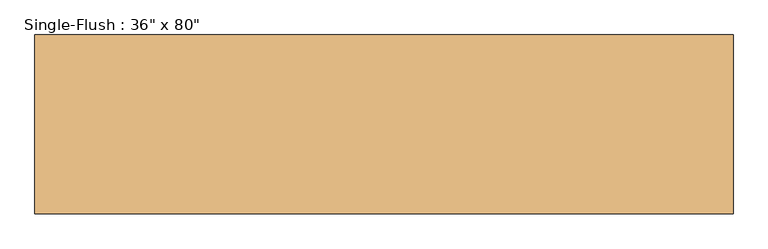
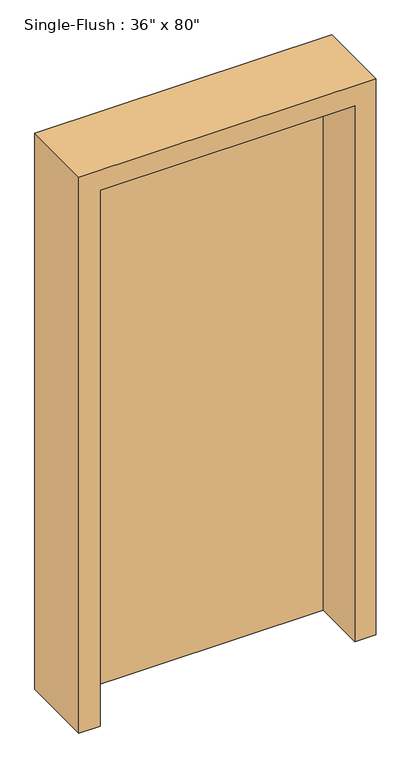
"""IFC4 building model written with IfcOpenShell, lengths in millimetres: door geometry."""

from ifc_helpers import new_model, si_unit, frame, origin, origin_with_axes, place, context, project, spatial, polyline, outline, extrude, source, transform, mapped, element, save


def door_dc32f4f0(model_context):
    return source(origin(), model_context, "Body", "SweptSolid", [
        extrude(outline(polyline([(2108.2, 533.4), (2108.2, -533.4), (0.0, -533.4), (0.0, -457.2), (2032.0, -457.2), (2032.0, 457.2), (0.0, 457.2), (0.0, 533.4), (2108.2, 533.4)])), frame((0.0, -136.525, 0.0), z_axis=(0.0, 1.0, 0.0), x_axis=(0.0, 0.0, 1.0)), (0.0, 0.0, 1.0), 273.05),
        extrude(outline(polyline([(457.2, 60.325), (-457.2, 60.325), (-457.2, 111.125), (457.2, 111.125), (457.2, 60.325)])), origin_with_axes(), (0.0, 0.0, 1.0), 2032.0),
    ])


if __name__ == "__main__":
    model = new_model("IFC4")
    model_context = context("Model", 3, world=origin())
    ifc_project = project(units=[si_unit("LENGTHUNIT", "METRE", prefix="MILLI")], contexts=[model_context])
    site = spatial("IfcSite", under=ifc_project)
    building = spatial("IfcBuilding", under=site)
    placement = place(None, origin())
    door_shape = door_dc32f4f0(model_context)
    element("IfcDoor", 1, ObjectType="Single-Flush : 36\" x 80\"", at=placement, inside=building, context=model_context, shape_type="MappedRepresentation", body=[
        mapped(door_shape, transform((0.0, 0.0, 0.0), x_axis=(1.0, 0.0, 0.0), y_axis=(0.0, 1.0, 0.0), z_axis=(0.0, 0.0, 1.0))),
    ])
    save(model, "model.ifc")

# Revit data of these elements
# Type "Single-Flush : 36\" x 80\""
#   Type Mark = "13"
#   Construction Type Id = "MDOOR"
#   Assembly Code = "C1020"
#   Analytic Construction = "Metal"
#   Thickness = 0' - 2"
#   Thermal Resistance (R) = 0.270117 (m²·K)/W
#   Heat Transfer Coefficient (U) = 3.7021 W/(m²·K)
#   Height = 6' - 8"
#   Trim Projection Ext = 0' - 1"
#   Trim Projection Int = 0' - 1"
#   Trim Width = 0' - 3"
#   Width = 3' - 0"
#   Door Material = INTERIOR GRADE ALUMINUM STOREFRONT W/ SAFETY GLAZING
#   Frame Material = INTERIOR GRADE ALUMINUM STOREFRONT W/ SAFETY GLAZING
#   Visual Light Transmittance = 0
#   Solar Heat Gain Coefficient = 0
#   Function = (empty or 0)
#   Wall Closure = (empty or 0)
# Element 1 (IfcDoor, "Single-Flush : 36\" x 80\"")
#   Materials on its faces: "INTERIOR GRADE ALUMINUM STOREFRONT W/ SAFETY GLAZING"
# Materials
#   "INTERIOR GRADE ALUMINUM STOREFRONT W/ SAFETY GLAZING": class "Metal", colour RGB 226 226 226, transparency 0, Description = "Aluminum 6061", Cost = 0
